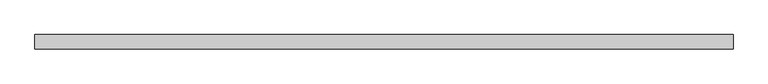
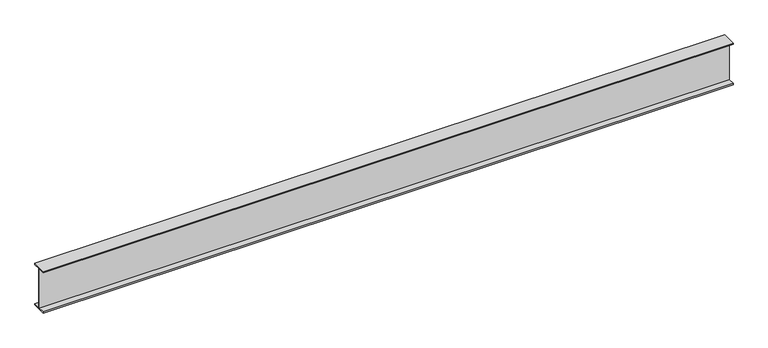
"""IFC4 building model written with IfcOpenShell, lengths in millimetres: proxy geometry, Generic Models 7:Generic Models 1:8:Generic Models 1:8 : Generic Models 7:Generic Models 1:337419:1 : Generic Models 7:Generic Models 1:8:Generic Models 1:8 : Generic Models 7:Generic Models 1:337419:315935."""

from ifc_helpers import new_model, si_unit, frame, origin, place, context, project, spatial, polyline, outline, extrude, source, transform, mapped, element, save


def generic_models_9655529d(model_context):
    return source(origin(), model_context, "Body", "SweptSolid", [
        extrude(outline(polyline([(-567904.3958012, 8538.8793773), (-567904.3958012, 8547.7693773), (-567802.5418012, 8547.7693773), (-567802.5418012, 8538.8793773), (-567850.4843012, 8538.8793773), (-567850.4843012, 8246.7793773), (-567802.5418012, 8246.7793773), (-567802.5418012, 8237.8893773), (-567904.3958012, 8237.8893773), (-567904.3958012, 8246.7793773), (-567856.4533012, 8246.7793773), (-567856.4533012, 8538.8793773), (-567904.3958012, 8538.8793773)])), frame((591306.0367242, 0.0, 0.0), z_axis=(1.0, 0.0, 0.0), x_axis=(0.0, 1.0, 0.0)), (0.0, 0.0, 1.0), 4876.8),
    ])


if __name__ == "__main__":
    model = new_model("IFC4")
    model_context = context("Model", 3, world=origin())
    ifc_project = project(units=[si_unit("LENGTHUNIT", "METRE", prefix="MILLI")], contexts=[model_context])
    site = spatial("IfcSite", under=ifc_project)
    building = spatial("IfcBuilding", under=site)
    placement = place(None, origin())
    generic_models_shape = generic_models_9655529d(model_context)
    element("IfcBuildingElementProxy", 1, Name="Generic Models 7:Generic Models 1:8:Generic Models 1:8 : Generic Models 7:Generic Models 1:337419:1 : Generic Models 7:Generic Models 1:8:Generic Models 1:8 : Generic Models 7:Generic Models 1:337419:315935", ObjectType="Generic Models 7:Generic Models 1:8:Generic Models 1:8 : Generic Models 7:Generic Models 1:337419:1 : Generic Models 7:Generic Models 1:8:Generic Models 1:8 : Generic Models 7:Generic Models 1:337419:315935", at=placement, inside=building, context=model_context, shape_type="MappedRepresentation", body=[
        mapped(generic_models_shape, transform((0.0, 0.0, 0.0), x_axis=(1.0, 0.0, 0.0), y_axis=(0.0, 1.0, 0.0), z_axis=(0.0, 0.0, 1.0))),
    ])
    save(model, "model.ifc")

# Revit data of these elements
# Type "Generic Models 7:Generic Models 1:8:Generic Models 1:8 : Generic Models 7:Generic Models 1:337419:1 : Generic Models 7:Generic Models 1:8:Generic Models 1:8 : Generic Models 7:Generic Models 1:337419:315935"
#   NameOverride = "Generic Models 7:Generic Models 1:8:Generic Models 1:8 : Generic Models 7:Generic Models 1:337419:315935"
#   ObjectTypeOverride = "Generic Models 1:8 : Generic Models 7:Generic Models 1:337419"
#   Reference = "Generic Models 1"
#   Tag = "315935"
# Element 1 (IfcBuildingElementProxy, "Generic Models 7:Generic Models 1:8:Generic Models 1:8 : Generic Models 7:Generic Models 1:337419:1 : Generic Models 7:Generic Models 1:8:Generic Models 1:8 : Generic Models 7:Generic Models 1:337419:315935")
#   Materials on its faces: "STRUCTURAL STEEL - SEE STRUCT. DWGS"
# Materials
#   "STRUCTURAL STEEL - SEE STRUCT. DWGS": class "Metal", colour RGB 189 187 185, transparency 0, Description = "Structural steel 50ksi", Cost = 0
